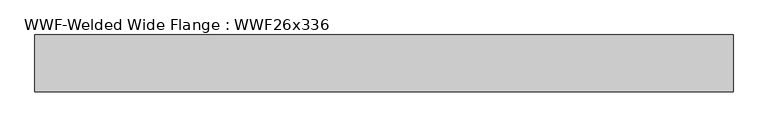
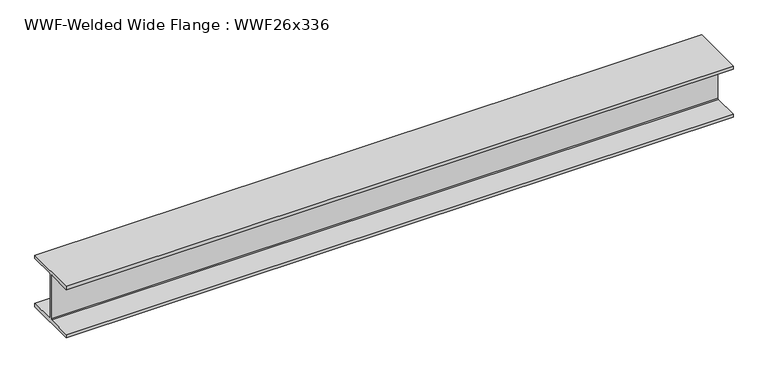
"""IFC4 building model written with IfcOpenShell, lengths in millimetres: beam geometry, WWF-Welded Wide Flange : WWF26x336."""

from ifc_helpers import new_model, si_unit, frame, origin, place, context, project, spatial, polyline, outline, extrude, source, transform, mapped, element, save


def wwf_welded_wide_flange_wwf26x336_ed01bac1(model_context):
    return source(origin(), model_context, "Body", "SweptSolid", [
        extrude(outline(polyline([(324.993, -284.988), (324.993, -324.993), (-324.993, -324.993), (-324.993, -284.988), (-20.6375, -284.988), (-9.9949, -274.3454), (-9.9949, 274.3454), (-20.6375, 284.988), (-324.993, 284.988), (-324.993, 324.993), (324.993, 324.993), (324.993, 284.988), (20.6375, 284.988), (9.9949, 274.3454), (9.9949, -274.3454), (20.6375, -284.988), (324.993, -284.988)])), frame((-3827.7582557, 0.0, 0.0), z_axis=(1.0, 0.0, 0.0), x_axis=(0.0, 1.0, 0.0)), (0.0, 0.0, 1.0), 7985.243261),
    ])


if __name__ == "__main__":
    model = new_model("IFC4")
    model_context = context("Model", 3, world=origin())
    ifc_project = project(units=[si_unit("LENGTHUNIT", "METRE", prefix="MILLI")], contexts=[model_context])
    site = spatial("IfcSite", under=ifc_project)
    building = spatial("IfcBuilding", under=site)
    placement = place(None, origin())
    wwf_welded_wide_flange_wwf26x336_shape = wwf_welded_wide_flange_wwf26x336_ed01bac1(model_context)
    element("IfcBeam", 1, ObjectType="WWF-Welded Wide Flange : WWF26x336", at=placement, inside=building, context=model_context, shape_type="MappedRepresentation", body=[
        mapped(wwf_welded_wide_flange_wwf26x336_shape, transform((0.0, 0.0, 0.0), x_axis=(1.0, 0.0, 0.0), y_axis=(0.0, 1.0, 0.0), z_axis=(0.0, 0.0, 1.0))),
    ])
    save(model, "model.ifc")

# Revit data of these elements
# Type "WWF-Welded Wide Flange : WWF26x336"
#   Assembly Code = "B10"
#   Nominal d = "12"
#   W = 336
#   Length [instance default] = 1524 mm
#   bf = 649.986 mm
#   d = 649.986 mm
#   k = 20.638 mm
#   tf = 40.005 mm
#   tw = 19.99 mm
#   A = 0.0635483 m²
#   Structural Material [instance default] = Steel ASTM A572
# Element 1 (IfcBeam, "WWF-Welded Wide Flange : WWF26x336")
#   Structural Material = Metal - Steel 43-275
#   Materials on its faces: "Metal - Steel 43-275"
# Materials
#   "Steel ASTM A572": class "Metal", colour RGB 247 247 247, transparency 0, Description = "Structural steel, high strength low alloy, ASTM - A572 - 50", Cost = 0
#   "Metal - Steel 43-275": class "Metal", colour RGB 247 247 247, transparency 0, Cost = 0
